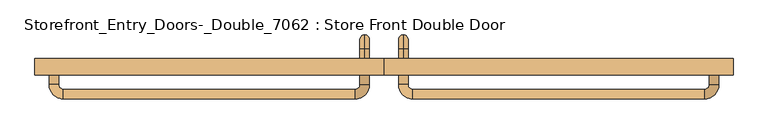
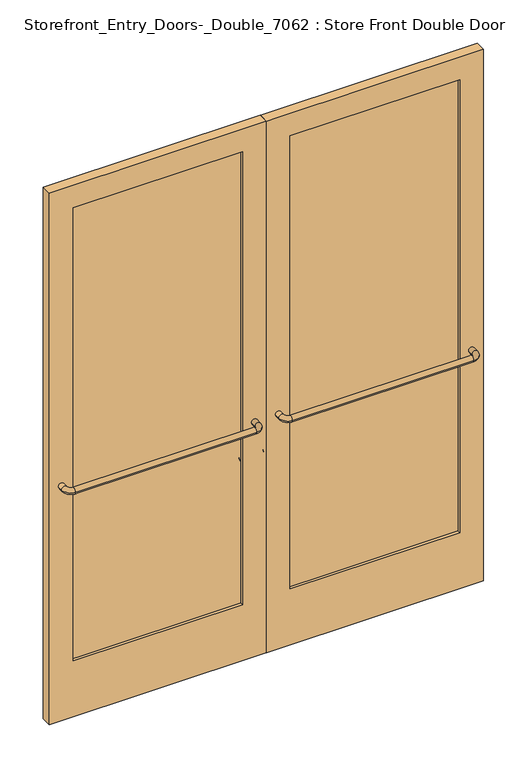
"""IFC4 building model written with IfcOpenShell, lengths in millimetres: door geometry, Storefront_Entry_Doors-_Double_7062 : Store Front Double Door."""

from ifc_helpers import new_model, si_unit, point, frame, origin, place, context, project, spatial, polyline, circle_curve, ellipse_curve, trimmed, outline, extrude, source, transform, mapped, element, save
from ifc_brep_helpers import plane_surface, cylinder_surface, revolved_surface, advanced_brep


def storefront_entry_doors_double_7062_store_front_double_door_b38478ba(model_context):
    return source(origin(), model_context, "Body", "SolidModel", [
        advanced_brep(
        [(51.59375, 50.8, 1079.5), (51.59375, 50.8, 1054.1), (51.59375, 76.2, 1079.5), (51.59375, 76.2, 1054.1), (51.59375, 88.9, 1041.4), (51.59375, 114.3, 1041.4), (51.59375, 114.3, 863.6), (51.59375, 88.9, 863.6), (51.59375, 76.2, 850.9), (51.59375, 76.2, 825.5), (51.59375, 50.8, 825.5), (51.59375, 50.8, 850.9)],
        [
            (0, 1, circle_curve(frame((51.59375, 50.8, 1066.8), z_axis=(0.0, -1.0, 0.0), x_axis=(0.0, 0.0, -1.0)), 12.7)),
            (1, 0, circle_curve(frame((51.59375, 50.8, 1066.8), z_axis=(0.0, -1.0, 0.0), x_axis=(0.0, 0.0, -1.0)), 12.7)),
            (0, 2),
            (2, 3, circle_curve(frame((51.59375, 76.2, 1066.8), z_axis=(0.0, -1.0, 0.0), x_axis=(0.0, 0.0, -1.0)), 12.7)),
            (3, 1),
            (3, 2, circle_curve(frame((51.59375, 76.2, 1066.8), z_axis=(0.0, -1.0, 0.0), x_axis=(0.0, 0.0, -1.0)), 12.7)),
            (4, 3, circle_curve(frame((51.59375, 76.2, 1041.4), z_axis=(1.0, 0.0, 0.0), x_axis=(0.0, 0.0, 1.0)), 12.7)),
            (2, 5, circle_curve(frame((51.59375, 76.2, 1041.4), z_axis=(-1.0, 0.0, 0.0), x_axis=(0.0, 0.0, 1.0)), 38.1)),
            (5, 4, circle_curve(frame((51.59375, 101.6, 1041.4), z_axis=(0.0, 0.0, 1.0), x_axis=(0.0, -1.0, 0.0)), 12.7)),
            (4, 5, circle_curve(frame((51.59375, 101.6, 1041.4), z_axis=(0.0, 0.0, 1.0), x_axis=(0.0, -1.0, 0.0)), 12.7)),
            (5, 6),
            (6, 7, circle_curve(frame((51.59375, 101.6, 863.6), z_axis=(0.0, 0.0, 1.0), x_axis=(0.0, -1.0, 0.0)), 12.7)),
            (7, 4),
            (7, 6, circle_curve(frame((51.59375, 101.6, 863.6), z_axis=(0.0, 0.0, 1.0), x_axis=(0.0, -1.0, 0.0)), 12.7)),
            (8, 7, circle_curve(frame((51.59375, 76.2, 863.6), z_axis=(1.0, 0.0, 0.0), x_axis=(0.0, 1.0, 0.0)), 12.7)),
            (6, 9, circle_curve(frame((51.59375, 76.2, 863.6), z_axis=(-1.0, 0.0, 0.0), x_axis=(0.0, 1.0, 0.0)), 38.1)),
            (9, 8, circle_curve(frame((51.59375, 76.2, 838.2), z_axis=(0.0, 1.0, 0.0), x_axis=(0.0, 0.0, 1.0)), 12.7)),
            (8, 9, circle_curve(frame((51.59375, 76.2, 838.2), z_axis=(0.0, 1.0, 0.0), x_axis=(0.0, 0.0, 1.0)), 12.7)),
            (10, 11, circle_curve(frame((51.59375, 50.8, 838.2), z_axis=(0.0, -1.0, 0.0), x_axis=(0.0, 0.0, 1.0)), 12.7)),
            (11, 10, circle_curve(frame((51.59375, 50.8, 838.2), z_axis=(0.0, -1.0, 0.0), x_axis=(0.0, 0.0, 1.0)), 12.7)),
            (9, 10),
            (11, 8),
        ],
        [
            plane_surface(frame((51.59375, 50.8, 1066.8), z_axis=(0.0, -1.0, 0.0), x_axis=(-1.0, 0.0, 0.0))),
            cylinder_surface(frame((51.59375, 50.8, 1066.8), z_axis=(0.0, -1.0, 0.0), x_axis=(0.0, 0.0, -1.0)), 12.7),
            revolved_surface(trimmed(ellipse_curve(frame((51.59375, 76.2, 1066.8), z_axis=(0.0, -1.0, 0.0), x_axis=(0.0, 0.0, -1.0)), 12.7, 12.7), [point((51.59375, 76.2, 1079.5))], [point((51.59375, 76.2, 1054.1))], True, "CARTESIAN"), (51.59375, 76.2, 1041.4), (-1.0, 0.0, 0.0)),
            revolved_surface(trimmed(ellipse_curve(frame((51.59375, 76.2, 1066.8), z_axis=(0.0, -1.0, 0.0), x_axis=(0.0, 0.0, -1.0)), 12.7, 12.7), [point((51.59375, 76.2, 1054.1))], [point((51.59375, 76.2, 1079.5))], True, "CARTESIAN"), (51.59375, 76.2, 1041.4), (-1.0, 0.0, 0.0)),
            cylinder_surface(frame((51.59375, 101.6, 1041.4), z_axis=(0.0, 0.0, 1.0), x_axis=(0.0, -1.0, 0.0)), 12.7),
            revolved_surface(trimmed(ellipse_curve(frame((51.59375, 101.6, 863.6), z_axis=(0.0, 0.0, 1.0), x_axis=(0.0, -1.0, 0.0)), 12.7, 12.7), [point((51.59375, 114.3, 863.6))], [point((51.59375, 88.9, 863.6))], True, "CARTESIAN"), (51.59375, 76.2, 863.6), (-1.0, 0.0, 0.0)),
            revolved_surface(trimmed(ellipse_curve(frame((51.59375, 101.6, 863.6), z_axis=(0.0, 0.0, 1.0), x_axis=(0.0, -1.0, 0.0)), 12.7, 12.7), [point((51.59375, 88.9, 863.6))], [point((51.59375, 114.3, 863.6))], True, "CARTESIAN"), (51.59375, 76.2, 863.6), (-1.0, 0.0, 0.0)),
            plane_surface(frame((51.59375, 50.8, 838.2), z_axis=(0.0, -1.0, 0.0), x_axis=(-1.0, 0.0, 0.0))),
            cylinder_surface(frame((51.59375, 76.2, 838.2), z_axis=(0.0, 1.0, 0.0), x_axis=(0.0, 0.0, 1.0)), 12.7),
        ],
        [
            (0, [[1, 2]]),
            (1, [[-1, 3, 4, 5]]),
            (1, [[-2, -5, 6, -3]]),
            (2, [[7, -4, 8, 9]]),
            (3, [[-8, -6, -7, 10]]),
            (4, [[-9, 11, 12, 13]]),
            (4, [[-10, -13, 14, -11]]),
            (5, [[15, -12, 16, 17]]),
            (6, [[-16, -14, -15, 18]]),
            (7, [[19, 20]]),
            (8, [[-17, 21, -20, 22]]),
            (8, [[-18, -22, -19, -21]]),
        ],
    ),
        advanced_brep(
        [(869.0428571, 6.35, 1066.8), (894.4428571, 6.35, 1066.8), (869.0428571, -19.05, 1066.8), (894.4428571, -19.05, 1066.8), (856.3428571, -57.15, 1066.8), (856.3428571, -31.75, 1066.8), (76.99375, -31.75, 1066.8), (76.99375, -57.15, 1066.8), (38.89375, -19.05, 1066.8), (64.29375, -19.05, 1066.8), (64.29375, 6.35, 1066.8), (38.89375, 6.35, 1066.8)],
        [
            (0, 1, circle_curve(frame((881.7428571, 6.35, 1066.8), z_axis=(0.0, 1.0, 0.0), x_axis=(1.0, 0.0, 0.0)), 12.7)),
            (1, 0, circle_curve(frame((881.7428571, 6.35, 1066.8), z_axis=(0.0, 1.0, 0.0), x_axis=(1.0, 0.0, 0.0)), 12.7)),
            (0, 2),
            (2, 3, circle_curve(frame((881.7428571, -19.05, 1066.8), z_axis=(0.0, 1.0, 0.0), x_axis=(1.0, 0.0, 0.0)), 12.7)),
            (3, 1),
            (3, 2, circle_curve(frame((881.7428571, -19.05, 1066.8), z_axis=(0.0, 1.0, 0.0), x_axis=(1.0, 0.0, 0.0)), 12.7)),
            (4, 3, circle_curve(frame((856.3428571, -19.05, 1066.8), z_axis=(0.0, 0.0, 1.0), x_axis=(1.0, 0.0, 0.0)), 38.1)),
            (2, 5, circle_curve(frame((856.3428571, -19.05, 1066.8), z_axis=(0.0, 0.0, -1.0), x_axis=(1.0, 0.0, 0.0)), 12.7)),
            (5, 4, circle_curve(frame((856.3428571, -44.45, 1066.8), z_axis=(1.0, 0.0, 0.0), x_axis=(0.0, -1.0, 0.0)), 12.7)),
            (4, 5, circle_curve(frame((856.3428571, -44.45, 1066.8), z_axis=(1.0, 0.0, 0.0), x_axis=(0.0, -1.0, 0.0)), 12.7)),
            (5, 6),
            (6, 7, circle_curve(frame((76.99375, -44.45, 1066.8), z_axis=(1.0, 0.0, 0.0), x_axis=(0.0, -1.0, 0.0)), 12.7)),
            (7, 4),
            (7, 6, circle_curve(frame((76.99375, -44.45, 1066.8), z_axis=(1.0, 0.0, 0.0), x_axis=(0.0, -1.0, 0.0)), 12.7)),
            (8, 7, circle_curve(frame((76.99375, -19.05, 1066.8), z_axis=(0.0, 0.0, 1.0), x_axis=(0.0, -1.0, 0.0)), 38.1)),
            (6, 9, circle_curve(frame((76.99375, -19.05, 1066.8), z_axis=(0.0, 0.0, -1.0), x_axis=(0.0, -1.0, 0.0)), 12.7)),
            (9, 8, circle_curve(frame((51.59375, -19.05, 1066.8), z_axis=(0.0, -1.0, 0.0), x_axis=(-1.0, 0.0, 0.0)), 12.7)),
            (8, 9, circle_curve(frame((51.59375, -19.05, 1066.8), z_axis=(0.0, -1.0, 0.0), x_axis=(-1.0, 0.0, 0.0)), 12.7)),
            (10, 11, circle_curve(frame((51.59375, 6.35, 1066.8), z_axis=(0.0, 1.0, 0.0), x_axis=(-1.0, 0.0, 0.0)), 12.7)),
            (11, 10, circle_curve(frame((51.59375, 6.35, 1066.8), z_axis=(0.0, 1.0, 0.0), x_axis=(-1.0, 0.0, 0.0)), 12.7)),
            (9, 10),
            (11, 8),
        ],
        [
            plane_surface(frame((881.7428571, 6.35, 1066.8), z_axis=(0.0, 1.0, 0.0), x_axis=(0.0, 0.0, 1.0))),
            cylinder_surface(frame((881.7428571, 6.35, 1066.8), z_axis=(0.0, 1.0, 0.0), x_axis=(1.0, 0.0, 0.0)), 12.7),
            revolved_surface(trimmed(ellipse_curve(frame((881.7428571, -19.05, 1066.8), z_axis=(0.0, 1.0, 0.0), x_axis=(1.0, 0.0, 0.0)), 12.7, 12.7), [point((869.0428571, -19.05, 1066.8))], [point((894.4428571, -19.05, 1066.8))], True, "CARTESIAN"), (856.3428571, -19.05, 1066.8), (0.0, 0.0, -1.0)),
            revolved_surface(trimmed(ellipse_curve(frame((881.7428571, -19.05, 1066.8), z_axis=(0.0, 1.0, 0.0), x_axis=(1.0, 0.0, 0.0)), 12.7, 12.7), [point((894.4428571, -19.05, 1066.8))], [point((869.0428571, -19.05, 1066.8))], True, "CARTESIAN"), (856.3428571, -19.05, 1066.8), (0.0, 0.0, -1.0)),
            cylinder_surface(frame((856.3428571, -44.45, 1066.8), z_axis=(1.0, 0.0, 0.0), x_axis=(0.0, -1.0, 0.0)), 12.7),
            revolved_surface(trimmed(ellipse_curve(frame((76.99375, -44.45, 1066.8), z_axis=(1.0, 0.0, 0.0), x_axis=(0.0, -1.0, 0.0)), 12.7, 12.7), [point((76.99375, -31.75, 1066.8))], [point((76.99375, -57.15, 1066.8))], True, "CARTESIAN"), (76.99375, -19.05, 1066.8), (0.0, 0.0, -1.0)),
            revolved_surface(trimmed(ellipse_curve(frame((76.99375, -44.45, 1066.8), z_axis=(1.0, 0.0, 0.0), x_axis=(0.0, -1.0, 0.0)), 12.7, 12.7), [point((76.99375, -57.15, 1066.8))], [point((76.99375, -31.75, 1066.8))], True, "CARTESIAN"), (76.99375, -19.05, 1066.8), (0.0, 0.0, -1.0)),
            plane_surface(frame((51.59375, 6.35, 1066.8), z_axis=(0.0, 1.0, 0.0), x_axis=(0.0, 0.0, 1.0))),
            cylinder_surface(frame((51.59375, -19.05, 1066.8), z_axis=(0.0, -1.0, 0.0), x_axis=(-1.0, 0.0, 0.0)), 12.7),
        ],
        [
            (0, [[1, 2]]),
            (1, [[-1, 3, 4, 5]]),
            (1, [[-2, -5, 6, -3]]),
            (2, [[7, -4, 8, 9]]),
            (3, [[-8, -6, -7, 10]]),
            (4, [[-9, 11, 12, 13]]),
            (4, [[-10, -13, 14, -11]]),
            (5, [[15, -12, 16, 17]]),
            (6, [[-16, -14, -15, 18]]),
            (7, [[19, 20]]),
            (8, [[-17, 21, -20, 22]]),
            (8, [[-18, -22, -19, -21]]),
        ],
    ),
        advanced_brep(
        [(-51.59375, 50.8, 1054.1), (-51.59375, 50.8, 1079.5), (-51.59375, 76.2, 1054.1), (-51.59375, 76.2, 1079.5), (-51.59375, 114.3, 1041.4), (-51.59375, 88.9, 1041.4), (-51.59375, 88.9, 863.6), (-51.59375, 114.3, 863.6), (-51.59375, 76.2, 825.5), (-51.59375, 76.2, 850.9), (-51.59375, 50.8, 850.9), (-51.59375, 50.8, 825.5)],
        [
            (0, 1, circle_curve(frame((-51.59375, 50.8, 1066.8), z_axis=(0.0, -1.0, 0.0), x_axis=(0.0, 0.0, 1.0)), 12.7)),
            (1, 0, circle_curve(frame((-51.59375, 50.8, 1066.8), z_axis=(0.0, -1.0, 0.0), x_axis=(0.0, 0.0, 1.0)), 12.7)),
            (0, 2),
            (2, 3, circle_curve(frame((-51.59375, 76.2, 1066.8), z_axis=(0.0, -1.0, 0.0), x_axis=(0.0, 0.0, 1.0)), 12.7)),
            (3, 1),
            (3, 2, circle_curve(frame((-51.59375, 76.2, 1066.8), z_axis=(0.0, -1.0, 0.0), x_axis=(0.0, 0.0, 1.0)), 12.7)),
            (4, 3, circle_curve(frame((-51.59375, 76.2, 1041.4), z_axis=(1.0, 0.0, 0.0), x_axis=(0.0, 0.0, 1.0)), 38.1)),
            (2, 5, circle_curve(frame((-51.59375, 76.2, 1041.4), z_axis=(-1.0, 0.0, 0.0), x_axis=(0.0, 0.0, 1.0)), 12.7)),
            (5, 4, circle_curve(frame((-51.59375, 101.6, 1041.4), z_axis=(0.0, 0.0, 1.0), x_axis=(0.0, 1.0, 0.0)), 12.7)),
            (4, 5, circle_curve(frame((-51.59375, 101.6, 1041.4), z_axis=(0.0, 0.0, 1.0), x_axis=(0.0, 1.0, 0.0)), 12.7)),
            (5, 6),
            (6, 7, circle_curve(frame((-51.59375, 101.6, 863.6), z_axis=(0.0, 0.0, 1.0), x_axis=(0.0, 1.0, 0.0)), 12.7)),
            (7, 4),
            (7, 6, circle_curve(frame((-51.59375, 101.6, 863.6), z_axis=(0.0, 0.0, 1.0), x_axis=(0.0, 1.0, 0.0)), 12.7)),
            (8, 7, circle_curve(frame((-51.59375, 76.2, 863.6), z_axis=(1.0, 0.0, 0.0), x_axis=(0.0, 1.0, 0.0)), 38.1)),
            (6, 9, circle_curve(frame((-51.59375, 76.2, 863.6), z_axis=(-1.0, 0.0, 0.0), x_axis=(0.0, 1.0, 0.0)), 12.7)),
            (9, 8, circle_curve(frame((-51.59375, 76.2, 838.2), z_axis=(0.0, 1.0, 0.0), x_axis=(0.0, 0.0, -1.0)), 12.7)),
            (8, 9, circle_curve(frame((-51.59375, 76.2, 838.2), z_axis=(0.0, 1.0, 0.0), x_axis=(0.0, 0.0, -1.0)), 12.7)),
            (10, 11, circle_curve(frame((-51.59375, 50.8, 838.2), z_axis=(0.0, -1.0, 0.0), x_axis=(0.0, 0.0, -1.0)), 12.7)),
            (11, 10, circle_curve(frame((-51.59375, 50.8, 838.2), z_axis=(0.0, -1.0, 0.0), x_axis=(0.0, 0.0, -1.0)), 12.7)),
            (9, 10),
            (11, 8),
        ],
        [
            plane_surface(frame((-51.59375, 50.8, 1066.8), z_axis=(0.0, -1.0, 0.0), x_axis=(1.0, 0.0, 0.0))),
            cylinder_surface(frame((-51.59375, 50.8, 1066.8), z_axis=(0.0, -1.0, 0.0), x_axis=(0.0, 0.0, 1.0)), 12.7),
            revolved_surface(trimmed(ellipse_curve(frame((-51.59375, 76.2, 1066.8), z_axis=(0.0, -1.0, 0.0), x_axis=(0.0, 0.0, 1.0)), 12.7, 12.7), [point((-51.59375, 76.2, 1054.1))], [point((-51.59375, 76.2, 1079.5))], True, "CARTESIAN"), (-51.59375, 76.2, 1041.4), (-1.0, 0.0, 0.0)),
            revolved_surface(trimmed(ellipse_curve(frame((-51.59375, 76.2, 1066.8), z_axis=(0.0, -1.0, 0.0), x_axis=(0.0, 0.0, 1.0)), 12.7, 12.7), [point((-51.59375, 76.2, 1079.5))], [point((-51.59375, 76.2, 1054.1))], True, "CARTESIAN"), (-51.59375, 76.2, 1041.4), (-1.0, 0.0, 0.0)),
            cylinder_surface(frame((-51.59375, 101.6, 1041.4), z_axis=(0.0, 0.0, 1.0), x_axis=(0.0, 1.0, 0.0)), 12.7),
            revolved_surface(trimmed(ellipse_curve(frame((-51.59375, 101.6, 863.6), z_axis=(0.0, 0.0, 1.0), x_axis=(0.0, 1.0, 0.0)), 12.7, 12.7), [point((-51.59375, 88.9, 863.6))], [point((-51.59375, 114.3, 863.6))], True, "CARTESIAN"), (-51.59375, 76.2, 863.6), (-1.0, 0.0, 0.0)),
            revolved_surface(trimmed(ellipse_curve(frame((-51.59375, 101.6, 863.6), z_axis=(0.0, 0.0, 1.0), x_axis=(0.0, 1.0, 0.0)), 12.7, 12.7), [point((-51.59375, 114.3, 863.6))], [point((-51.59375, 88.9, 863.6))], True, "CARTESIAN"), (-51.59375, 76.2, 863.6), (-1.0, 0.0, 0.0)),
            plane_surface(frame((-51.59375, 50.8, 838.2), z_axis=(0.0, -1.0, 0.0), x_axis=(1.0, 0.0, 0.0))),
            cylinder_surface(frame((-51.59375, 76.2, 838.2), z_axis=(0.0, 1.0, 0.0), x_axis=(0.0, 0.0, -1.0)), 12.7),
        ],
        [
            (0, [[1, 2]]),
            (1, [[-1, 3, 4, 5]]),
            (1, [[-2, -5, 6, -3]]),
            (2, [[7, -4, 8, 9]]),
            (3, [[-8, -6, -7, 10]]),
            (4, [[-9, 11, 12, 13]]),
            (4, [[-10, -13, 14, -11]]),
            (5, [[15, -12, 16, 17]]),
            (6, [[-16, -14, -15, 18]]),
            (7, [[19, 20]]),
            (8, [[-17, 21, -20, 22]]),
            (8, [[-18, -22, -19, -21]]),
        ],
    ),
        advanced_brep(
        [(-64.29375, 6.35, 1066.8), (-38.89375, 6.35, 1066.8), (-64.29375, -19.05, 1066.8), (-38.89375, -19.05, 1066.8), (-76.99375, -57.15, 1066.8), (-76.99375, -31.75, 1066.8), (-856.3428571, -31.75, 1066.8), (-856.3428571, -57.15, 1066.8), (-894.4428571, -19.05, 1066.8), (-869.0428571, -19.05, 1066.8), (-869.0428571, 6.35, 1066.8), (-894.4428571, 6.35, 1066.8)],
        [
            (0, 1, circle_curve(frame((-51.59375, 6.35, 1066.8), z_axis=(0.0, 1.0, 0.0), x_axis=(1.0, 0.0, 0.0)), 12.7)),
            (1, 0, circle_curve(frame((-51.59375, 6.35, 1066.8), z_axis=(0.0, 1.0, 0.0), x_axis=(1.0, 0.0, 0.0)), 12.7)),
            (0, 2),
            (2, 3, circle_curve(frame((-51.59375, -19.05, 1066.8), z_axis=(0.0, 1.0, 0.0), x_axis=(1.0, 0.0, 0.0)), 12.7)),
            (3, 1),
            (3, 2, circle_curve(frame((-51.59375, -19.05, 1066.8), z_axis=(0.0, 1.0, 0.0), x_axis=(1.0, 0.0, 0.0)), 12.7)),
            (4, 3, circle_curve(frame((-76.99375, -19.05, 1066.8), z_axis=(0.0, 0.0, 1.0), x_axis=(1.0, 0.0, 0.0)), 38.1)),
            (2, 5, circle_curve(frame((-76.99375, -19.05, 1066.8), z_axis=(0.0, 0.0, -1.0), x_axis=(1.0, 0.0, 0.0)), 12.7)),
            (5, 4, circle_curve(frame((-76.99375, -44.45, 1066.8), z_axis=(1.0, 0.0, 0.0), x_axis=(0.0, -1.0, 0.0)), 12.7)),
            (4, 5, circle_curve(frame((-76.99375, -44.45, 1066.8), z_axis=(1.0, 0.0, 0.0), x_axis=(0.0, -1.0, 0.0)), 12.7)),
            (5, 6),
            (6, 7, circle_curve(frame((-856.3428571, -44.45, 1066.8), z_axis=(1.0, 0.0, 0.0), x_axis=(0.0, -1.0, 0.0)), 12.7)),
            (7, 4),
            (7, 6, circle_curve(frame((-856.3428571, -44.45, 1066.8), z_axis=(1.0, 0.0, 0.0), x_axis=(0.0, -1.0, 0.0)), 12.7)),
            (8, 7, circle_curve(frame((-856.3428571, -19.05, 1066.8), z_axis=(0.0, 0.0, 1.0), x_axis=(0.0, -1.0, 0.0)), 38.1)),
            (6, 9, circle_curve(frame((-856.3428571, -19.05, 1066.8), z_axis=(0.0, 0.0, -1.0), x_axis=(0.0, -1.0, 0.0)), 12.7)),
            (9, 8, circle_curve(frame((-881.7428571, -19.05, 1066.8), z_axis=(0.0, -1.0, 0.0), x_axis=(-1.0, 0.0, 0.0)), 12.7)),
            (8, 9, circle_curve(frame((-881.7428571, -19.05, 1066.8), z_axis=(0.0, -1.0, 0.0), x_axis=(-1.0, 0.0, 0.0)), 12.7)),
            (10, 11, circle_curve(frame((-881.7428571, 6.35, 1066.8), z_axis=(0.0, 1.0, 0.0), x_axis=(-1.0, 0.0, 0.0)), 12.7)),
            (11, 10, circle_curve(frame((-881.7428571, 6.35, 1066.8), z_axis=(0.0, 1.0, 0.0), x_axis=(-1.0, 0.0, 0.0)), 12.7)),
            (9, 10),
            (11, 8),
        ],
        [
            plane_surface(frame((-51.59375, 6.35, 1066.8), z_axis=(0.0, 1.0, 0.0), x_axis=(0.0, 0.0, 1.0))),
            cylinder_surface(frame((-51.59375, 6.35, 1066.8), z_axis=(0.0, 1.0, 0.0), x_axis=(1.0, 0.0, 0.0)), 12.7),
            revolved_surface(trimmed(ellipse_curve(frame((-51.59375, -19.05, 1066.8), z_axis=(0.0, 1.0, 0.0), x_axis=(1.0, 0.0, 0.0)), 12.7, 12.7), [point((-64.29375, -19.05, 1066.8))], [point((-38.89375, -19.05, 1066.8))], True, "CARTESIAN"), (-76.99375, -19.05, 1066.8), (0.0, 0.0, -1.0)),
            revolved_surface(trimmed(ellipse_curve(frame((-51.59375, -19.05, 1066.8), z_axis=(0.0, 1.0, 0.0), x_axis=(1.0, 0.0, 0.0)), 12.7, 12.7), [point((-38.89375, -19.05, 1066.8))], [point((-64.29375, -19.05, 1066.8))], True, "CARTESIAN"), (-76.99375, -19.05, 1066.8), (0.0, 0.0, -1.0)),
            cylinder_surface(frame((-76.99375, -44.45, 1066.8), z_axis=(1.0, 0.0, 0.0), x_axis=(0.0, -1.0, 0.0)), 12.7),
            revolved_surface(trimmed(ellipse_curve(frame((-856.3428571, -44.45, 1066.8), z_axis=(1.0, 0.0, 0.0), x_axis=(0.0, -1.0, 0.0)), 12.7, 12.7), [point((-856.3428571, -31.75, 1066.8))], [point((-856.3428571, -57.15, 1066.8))], True, "CARTESIAN"), (-856.3428571, -19.05, 1066.8), (0.0, 0.0, -1.0)),
            revolved_surface(trimmed(ellipse_curve(frame((-856.3428571, -44.45, 1066.8), z_axis=(1.0, 0.0, 0.0), x_axis=(0.0, -1.0, 0.0)), 12.7, 12.7), [point((-856.3428571, -57.15, 1066.8))], [point((-856.3428571, -31.75, 1066.8))], True, "CARTESIAN"), (-856.3428571, -19.05, 1066.8), (0.0, 0.0, -1.0)),
            plane_surface(frame((-881.7428571, 6.35, 1066.8), z_axis=(0.0, 1.0, 0.0), x_axis=(0.0, 0.0, 1.0))),
            cylinder_surface(frame((-881.7428571, -19.05, 1066.8), z_axis=(0.0, -1.0, 0.0), x_axis=(-1.0, 0.0, 0.0)), 12.7),
        ],
        [
            (0, [[1, 2]]),
            (1, [[-1, 3, 4, 5]]),
            (1, [[-2, -5, 6, -3]]),
            (2, [[7, -4, 8, 9]]),
            (3, [[-8, -6, -7, 10]]),
            (4, [[-9, 11, 12, 13]]),
            (4, [[-10, -13, 14, -11]]),
            (5, [[15, -12, 16, 17]]),
            (6, [[-16, -14, -15, 18]]),
            (7, [[19, 20]]),
            (8, [[-17, 21, -20, 22]]),
            (8, [[-18, -22, -19, -21]]),
        ],
    ),
        extrude(outline(polyline([(830.9428571, 19.05), (102.39375, 19.05), (102.39375, 38.1), (830.9428571, 38.1), (830.9428571, 19.05)])), frame((0.0, 0.0, 254.0), z_axis=(0.0, 0.0, 1.0), x_axis=(1.0, 0.0, 0.0)), (0.0, 0.0, 1.0), 2057.4),
        extrude(outline(polyline([(-102.39375, 19.05), (-830.9428571, 19.05), (-830.9428571, 38.1), (-102.39375, 38.1), (-102.39375, 19.05)])), frame((0.0, 0.0, 254.0), z_axis=(0.0, 0.0, 1.0), x_axis=(1.0, 0.0, 0.0)), (0.0, 0.0, 1.0), 2057.4),
        extrude(outline(polyline([(2413.0, 0.79375), (0.0, 0.79375), (0.0, 932.5428571), (2413.0, 932.5428571), (2413.0, 0.79375)]), holes=[polyline([(2311.4, 102.39375), (2311.4, 830.9428571), (254.0, 830.9428571), (254.0, 102.39375), (2311.4, 102.39375)])]), frame((0.0, 6.35, 0.0), z_axis=(0.0, 1.0, 0.0), x_axis=(0.0, 0.0, 1.0)), (0.0, 0.0, 1.0), 44.45),
        extrude(outline(polyline([(2413.0, -0.79375), (2413.0, -932.5428571), (0.0, -932.5428571), (0.0, -0.79375), (2413.0, -0.79375)]), holes=[polyline([(2311.4, -830.9428571), (2311.4, -102.39375), (254.0, -102.39375), (254.0, -830.9428571), (2311.4, -830.9428571)])]), frame((0.0, 6.35, 0.0), z_axis=(0.0, 1.0, 0.0), x_axis=(0.0, 0.0, 1.0)), (0.0, 0.0, 1.0), 44.45),
    ])


if __name__ == "__main__":
    model = new_model("IFC4")
    model_context = context("Model", 3, world=origin())
    ifc_project = project(units=[si_unit("LENGTHUNIT", "METRE", prefix="MILLI")], contexts=[model_context])
    site = spatial("IfcSite", under=ifc_project)
    building = spatial("IfcBuilding", under=site)
    placement = place(None, origin())
    storefront_entry_doors_double_7062_store_front_double_door_shape = storefront_entry_doors_double_7062_store_front_double_door_b38478ba(model_context)
    element("IfcDoor", 1, ObjectType="Storefront_Entry_Doors-_Double_7062 : Store Front Double Door", at=placement, inside=building, context=model_context, shape_type="MappedRepresentation", body=[
        mapped(storefront_entry_doors_double_7062_store_front_double_door_shape, transform((0.0, 0.0, 0.0), x_axis=(1.0, 0.0, 0.0), y_axis=(0.0, 1.0, 0.0), z_axis=(0.0, 0.0, 1.0))),
    ])
    save(model, "model.ifc")

# Revit data of these elements
# Type "Storefront_Entry_Doors-_Double_7062 : Store Front Double Door"
#   Type Mark = "20"
#   Assembly Code = "B2030110"
#   Top Rail = 0' - 4"
#   Side Rail = 0' - 4"
#   Rail Height AFF = 3' - 6"
#   Offset = 0' - 2"
#   Bottom Rail Width = 0' - 10"
#   Material = Metal - Aluminum
#   Glazing Material = Glass
#   Function = (empty or 0)
# Element 1 (IfcDoor, "Storefront_Entry_Doors-_Double_7062 : Store Front Double Door")
#   Materials on its faces: "Metal - Aluminum", "Glass"
# Materials
#   "Metal - Aluminum": class "Metal", colour RGB 247 247 247, transparency 0
#   "Glass": class "Glass", colour RGB 218 227 224, transparency 0.85, Description = "Soda Lime Glass", Cost = 0
